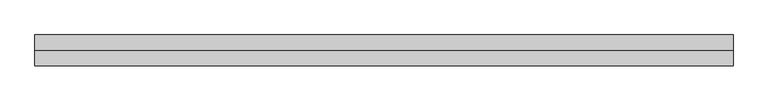
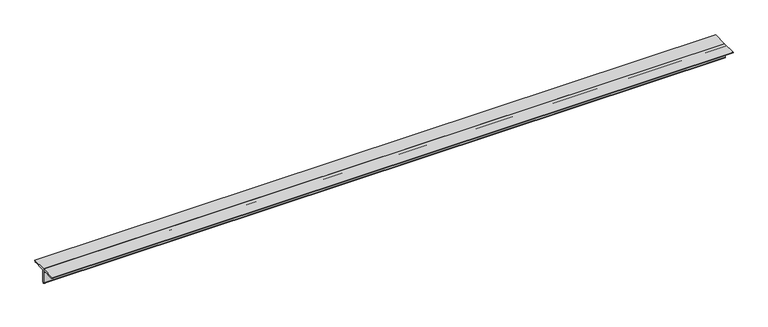
"""IFC4 building model written with IfcOpenShell, lengths in millimetres: member geometry, 0123_Steel Framing_2Ls-KSD3502 : H_SB_AR_S03_2Ls-130x130x12_HBR1."""

import ifcopenshell
import ifcopenshell.guid

model = None  # the IFC model being written
_history = None  # IfcOwnerHistory: only IFC2X3 demands one
_inside = {}  # id of a spatial element -> (the spatial element, [elements in it])
_under = {}  # id of a project, library or spatial element -> (it, [spatial elements below it])
_declared = {}  # id of a project -> (the project, [libraries it declares])
_typed = {}  # id of a type object -> (the type object, [elements of that type])
_made_of = {}  # id of a material, layer set ... -> (it, [elements and type objects made of it])


def new_model(schema):
    """Start an empty IFC model of exactly this schema.

    Asked for "IFC4X3", IfcOpenShell would pick the latest addendum, in which some entities
    have other attributes; the version numbers below select the first issue.
    IFC2X3 requires an IfcOwnerHistory on every rooted entity: one is made here for all.
    """
    global model, _history
    if schema == "IFC4X3":
        model = ifcopenshell.file(schema_version=(4, 3, 0, 0))
    else:
        model = ifcopenshell.file(schema=schema)
    _inside.clear()
    _under.clear()
    _declared.clear()
    _typed.clear()
    _made_of.clear()
    _history = None
    if model.schema == "IFC2X3":
        org = make("IfcOrganization", Name="unknown")
        user = make(
            "IfcPersonAndOrganization",
            ThePerson=make("IfcPerson", FamilyName="unknown"),
            TheOrganization=org,
        )
        app = make(
            "IfcApplication",
            ApplicationDeveloper=org,
            Version="unknown",
            ApplicationFullName="unknown",
            ApplicationIdentifier="unknown",
        )
        _history = make(
            "IfcOwnerHistory",
            OwningUser=user,
            OwningApplication=app,
            ChangeAction="ADDED",
            CreationDate=0,
        )
    return model


def make(cls, **values):
    """One entity of the class cls with the attributes given. An attribute that is None is left unset."""
    return model.create_entity(
        cls, **{name: value for name, value in values.items() if value is not None}
    )


def rooted(cls, **values):
    """An entity with a GlobalId (a new one), such as an element, a storey or a relation."""
    return make(cls, GlobalId=ifcopenshell.guid.new(), OwnerHistory=_history, **values)


def si_unit(unit_type, name, prefix=None):
    """IfcSIUnit, for example si_unit("LENGTHUNIT", "METRE", prefix="MILLI")."""
    return make("IfcSIUnit", UnitType=unit_type, Prefix=prefix, Name=name)


def assignment(units):
    """IfcUnitAssignment: the units of a project."""
    return None if units is None else make("IfcUnitAssignment", Units=units)


def point(xyz):
    """IfcCartesianPoint."""
    return None if xyz is None else make("IfcCartesianPoint", Coordinates=xyz)


def direction(xyz):
    """IfcDirection."""
    return None if xyz is None else make("IfcDirection", DirectionRatios=xyz)


def frame(location, z_axis=None, x_axis=None):
    """IfcAxis2Placement3D, a coordinate frame: its origin and axes. An axis left out is left unset."""
    return make(
        "IfcAxis2Placement3D",
        Location=point(location),
        Axis=direction(z_axis),
        RefDirection=direction(x_axis),
    )


def frame_2d(location, x_axis=None):
    """IfcAxis2Placement2D, a coordinate frame in the plane: its origin and x axis."""
    return make(
        "IfcAxis2Placement2D", Location=point(location), RefDirection=direction(x_axis)
    )


def origin():
    """The frame at (0, 0, 0) with its axes left unset."""
    return frame((0.0, 0.0, 0.0))


def place(relative_to, where):
    """IfcLocalPlacement: puts the frame where relative to a parent placement (None: the world)."""
    return make(
        "IfcLocalPlacement", PlacementRelTo=relative_to, RelativePlacement=where
    )


def context(
    kind, dimensions, precision=None, world=None, true_north=None, identifier=None
):
    """IfcGeometricRepresentationContext, for example the 3D "Model" context."""
    return make(
        "IfcGeometricRepresentationContext",
        ContextIdentifier=identifier,
        ContextType=kind,
        CoordinateSpaceDimension=dimensions,
        Precision=precision,
        WorldCoordinateSystem=world,
        TrueNorth=true_north,
    )


def project(units=None, contexts=None):
    """IfcProject with its units and contexts."""
    return rooted(
        "IfcProject",
        Name="project",
        RepresentationContexts=contexts,
        UnitsInContext=assignment(units),
    )


def spatial(cls, under=None, at=None, **own):
    """A site, building, storey or space (cls), placed at a placement, below another one or the project."""
    s = rooted(cls, ObjectPlacement=at, **own)
    if under is not None:
        _under.setdefault(under.id(), (under, []))[1].append(s)
    return s


def polyline(points):
    """IfcPolyline through the points."""
    return make("IfcPolyline", Points=[point(p) for p in points])


def circle_curve(where, radius):
    """IfcCircle in the frame where."""
    return make("IfcCircle", Position=where, Radius=radius)


def trimmed(basis, trim1, trim2, sense, master):
    """IfcTrimmedCurve: the piece of a basis curve between two trims."""
    return make(
        "IfcTrimmedCurve",
        BasisCurve=basis,
        Trim1=trim1,
        Trim2=trim2,
        SenseAgreement=sense,
        MasterRepresentation=master,
    )


def segment(curve, same_sense, transition):
    """IfcCompositeCurveSegment."""
    return make(
        "IfcCompositeCurveSegment",
        Transition=transition,
        SameSense=same_sense,
        ParentCurve=curve,
    )


def composite_curve(segments, self_intersect=None):
    """IfcCompositeCurve: segments joined end to end."""
    return make("IfcCompositeCurve", Segments=segments, SelfIntersect=self_intersect)


def outline(outer, holes=None, kind="AREA"):
    """IfcArbitraryClosedProfileDef: a profile drawn as a closed curve; with holes, ...WithVoids."""
    if holes is None:
        return make("IfcArbitraryClosedProfileDef", ProfileType=kind, OuterCurve=outer)
    return make(
        "IfcArbitraryProfileDefWithVoids",
        ProfileType=kind,
        OuterCurve=outer,
        InnerCurves=holes,
    )


def extrude(swept, where, along, depth):
    """IfcExtrudedAreaSolid: the profile swept, set in the frame where, extruded along a direction by depth."""
    return make(
        "IfcExtrudedAreaSolid",
        SweptArea=swept,
        Position=where,
        ExtrudedDirection=direction(along),
        Depth=depth,
    )


def shape(context_of_items, identifier, shape_type, items):
    """IfcShapeRepresentation: the items that make up one representation, for example the "Body"."""
    return make(
        "IfcShapeRepresentation",
        ContextOfItems=context_of_items,
        RepresentationIdentifier=identifier,
        RepresentationType=shape_type,
        Items=items,
    )


def source(mapping_origin, context_of_items, identifier, shape_type, items):
    """IfcRepresentationMap: a shape defined once, which mapped items show again and again."""
    return make(
        "IfcRepresentationMap",
        MappingOrigin=mapping_origin,
        MappedRepresentation=shape(context_of_items, identifier, shape_type, items),
    )


def transform(
    local_origin,
    x_axis=None,
    y_axis=None,
    z_axis=None,
    scale=None,
    scale2=None,
    scale3=None,
    uniform=True,
):
    """IfcCartesianTransformationOperator3D, or its non-uniform kind. x_axis, y_axis, z_axis: its Axis1, 2, 3."""
    if uniform:
        return make(
            "IfcCartesianTransformationOperator3D",
            Axis1=direction(x_axis),
            Axis2=direction(y_axis),
            LocalOrigin=point(local_origin),
            Scale=scale,
            Axis3=direction(z_axis),
        )
    return make(
        "IfcCartesianTransformationOperator3DnonUniform",
        Axis1=direction(x_axis),
        Axis2=direction(y_axis),
        LocalOrigin=point(local_origin),
        Scale=scale,
        Axis3=direction(z_axis),
        Scale2=scale2,
        Scale3=scale3,
    )


def mapped(mapping_source, mapping_target):
    """IfcMappedItem: shows the shape of a source again, moved by a transform."""
    return make(
        "IfcMappedItem", MappingSource=mapping_source, MappingTarget=mapping_target
    )


def made_of(thing, what):
    """Note that an element or type object is made of a material, layer set ...; save() writes the relation."""
    if what is not None:
        _made_of.setdefault(what.id(), (what, []))[1].append(thing)
    return thing


def element(
    cls,
    number,
    at=None,
    inside=None,
    cuts=None,
    type_object=None,
    material=None,
    context=None,
    identifier="Body",
    shape_type=None,
    held_by="IfcProductDefinitionShape",
    body=None,
    shapes=None,
    **own,
):
    """One element of the class cls, such as IfcWall. Its Tag is "e" and its number.

    at: its placement. inside: the storey or other place that contains it. cuts: it is an
    opening in that element (IfcRelVoidsElement). A single representation is given by context,
    identifier, shape_type and body (its items); several are given by shapes. held_by: the class
    of the entity that holds the representations. save() writes the other relations.
    """
    e = rooted(cls, Tag="e%d" % number, ObjectPlacement=at, **own)
    if body is not None:
        shapes = [shape(context, identifier, shape_type, body)]
    if shapes is not None:
        e.Representation = make(held_by, Representations=shapes)
    if inside is not None:
        _inside.setdefault(inside.id(), (inside, []))[1].append(e)
    if cuts is not None:
        rooted(
            "IfcRelVoidsElement", RelatingBuildingElement=cuts, RelatedOpeningElement=e
        )
    if type_object is not None:
        _typed.setdefault(type_object.id(), (type_object, []))[1].append(e)
    return made_of(e, material)


def aggregate(whole, parts):
    """IfcRelAggregates: a whole, such as a stair, and the parts it consists of."""
    return rooted("IfcRelAggregates", RelatingObject=whole, RelatedObjects=parts)


def save(model, path):
    """Write the relations noted so far, then the file.

    IfcRelAggregates (storeys below a building ...), IfcRelContainedInSpatialStructure (elements
    in a storey), IfcRelDefinesByType, IfcRelAssociatesMaterial and IfcRelDeclares: one each for
    every whole, place, type object, material and project.
    """
    for whole, parts in _under.values():
        aggregate(whole, parts)
    for where, things in _inside.values():
        rooted(
            "IfcRelContainedInSpatialStructure",
            RelatedElements=things,
            RelatingStructure=where,
        )
    for kind, things in _typed.values():
        rooted("IfcRelDefinesByType", RelatedObjects=things, RelatingType=kind)
    for what, things in _made_of.values():
        rooted("IfcRelAssociatesMaterial", RelatedObjects=things, RelatingMaterial=what)
    for by, libraries in _declared.values():
        rooted("IfcRelDeclares", RelatingContext=by, RelatedDefinitions=libraries)
    model.write(path)


def member_5d0c7e09(model_context):
    return source(origin(), model_context, "Body", "SweptSolid", [
        extrude(outline(composite_curve([segment(polyline([(0.0, 36.4), (130.0, 36.4)]), True, "CONTINUOUS"), segment(trimmed(circle_curve(frame_2d((118.0, 36.4)), 12.0), [point((130.0, 36.4))], [point((118.0, 24.4))], False, "CARTESIAN"), True, "CONTINUOUS"), segment(polyline([(118.0, 24.4), (24.0, 24.4)]), True, "CONTINUOUS"), segment(trimmed(circle_curve(frame_2d((24.0, 12.4)), 12.0), [point((24.0, 24.4))], [point((12.0, 12.4))], True, "CARTESIAN"), True, "CONTINUOUS"), segment(polyline([(12.0, 12.4), (12.0, -81.6)]), True, "CONTINUOUS"), segment(trimmed(circle_curve(frame_2d((0.0, -81.6)), 12.0), [point((12.0, -81.6))], [point((0.0, -93.6))], False, "CARTESIAN"), True, "CONTINUOUS"), segment(polyline([(0.0, -93.6), (0.0, 36.4)]), True, "CONTINUOUS")], self_intersect=False)), frame((-2943.7629586, 0.0, 0.0), z_axis=(1.0, 0.0, 0.0), x_axis=(0.0, 1.0, 0.0)), (0.0, 0.0, 1.0), 5889.8945249),
        extrude(outline(composite_curve([segment(polyline([(0.0, 36.4), (0.0, -93.6)]), True, "CONTINUOUS"), segment(trimmed(circle_curve(frame_2d((0.0, -81.6)), 12.0), [point((0.0, -93.6))], [point((-12.0, -81.6))], False, "CARTESIAN"), True, "CONTINUOUS"), segment(polyline([(-12.0, -81.6), (-12.0, 12.4)]), True, "CONTINUOUS"), segment(trimmed(circle_curve(frame_2d((-24.0, 12.4)), 12.0), [point((-12.0, 12.4))], [point((-24.0, 24.4))], True, "CARTESIAN"), True, "CONTINUOUS"), segment(polyline([(-24.0, 24.4), (-118.0, 24.4)]), True, "CONTINUOUS"), segment(trimmed(circle_curve(frame_2d((-118.0, 36.4)), 12.0), [point((-118.0, 24.4))], [point((-130.0, 36.4))], False, "CARTESIAN"), True, "CONTINUOUS"), segment(polyline([(-130.0, 36.4), (0.0, 36.4)]), True, "CONTINUOUS")], self_intersect=False)), frame((-2943.7629586, 0.0, 0.0), z_axis=(1.0, 0.0, 0.0), x_axis=(0.0, 1.0, 0.0)), (0.0, 0.0, 1.0), 5889.8945249),
    ])


if __name__ == "__main__":
    model = new_model("IFC4")
    model_context = context("Model", 3, world=origin())
    ifc_project = project(units=[si_unit("LENGTHUNIT", "METRE", prefix="MILLI")], contexts=[model_context])
    site = spatial("IfcSite", under=ifc_project)
    building = spatial("IfcBuilding", under=site)
    placement = place(None, origin())
    member_shape = member_5d0c7e09(model_context)
    element("IfcMember", 1, ObjectType="0123_Steel Framing_2Ls-KSD3502 : H_SB_AR_S03_2Ls-130x130x12_HBR1", at=placement, inside=building, context=model_context, shape_type="MappedRepresentation", body=[
        mapped(member_shape, transform((0.0, 0.0, 0.0), x_axis=(1.0, 0.0, 0.0), y_axis=(0.0, 1.0, 0.0), z_axis=(0.0, 0.0, 1.0))),
    ])
    save(model, "model.ifc")

# Revit data of these elements
# Type "0123_Steel Framing_2Ls-KSD3502 : H_SB_AR_S03_2Ls-130x130x12_HBR1"
#   Type Mark = "HBR1"
#   Assembly Code = "B10"
#   Legs = "SLBB"
#   W = 8.97
#   Perimeter = 1.04 m²/m
#   Nominal Weight = 46.80 kgf/m
#   Length [instance default] = 1000 mm
#   Space = 0 mm
#   b = 130 mm
#   d = 130 mm
#   t = 12 mm
#   y = 36.4 mm
#   A = 0.005952 m²
#   Structural Material [instance default] = Steel ASTM A36
# Element 1 (IfcMember, "0123_Steel Framing_2Ls-KSD3502 : H_SB_AR_S03_2Ls-130x130x12_HBR1")
#   Materials on its faces: "Steel ASTM A36"
# Materials
#   "Steel ASTM A36": class "Metal", colour RGB 199 199 199, transparency 0, Description = "Structural steel, ASTM A36 Grade B, mill finish", Cost = 0
